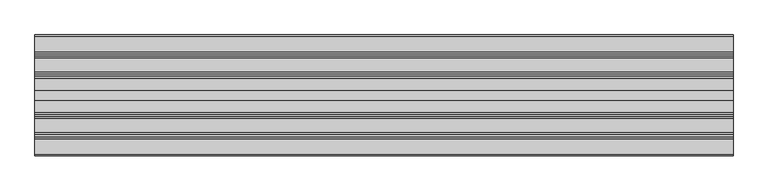
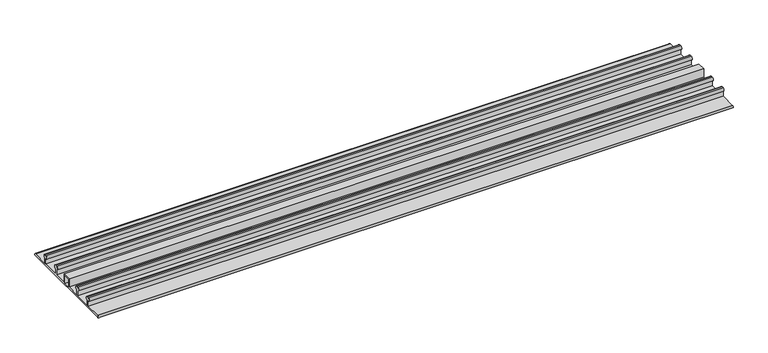
"""IFC4 building model written with IfcOpenShell, lengths in millimetres: proxy geometry, TN_ПВХ_ТПО_Гидрошпонка ТехноНИКОЛЬ : ПВХ Гидрошпонка ТехноНИКОЛЬ EM-260/20."""

from ifc_helpers import new_model, si_unit, point, frame, frame_2d, origin, place, context, project, spatial, polyline, circle_curve, trimmed, segment, composite_curve, outline, extrude, source, transform, mapped, element, save


def specialty_equipment_cb169843(model_context):
    return source(origin(), model_context, "Body", "SweptSolid", [
        extrude(outline(composite_curve([segment(polyline([(127.5, 0.0), (-127.5, 0.0)]), True, "CONTINUOUS"), segment(trimmed(circle_curve(frame_2d((-127.5, 2.5)), 2.5), [point((-127.5, 0.0))], [point((-127.5, 5.0))], False, "CARTESIAN"), True, "CONTINUOUS"), segment(polyline([(-127.5, 5.0), (-88.7123259, 5.0), (-88.7123259, 18.0)]), True, "CONTINUOUS"), segment(trimmed(circle_curve(frame_2d((-88.7123259, 22.0)), 4.0), [point((-88.7123259, 18.0))], [point((-88.7123259, 26.0))], False, "CARTESIAN"), True, "CONTINUOUS"), segment(polyline([(-88.7123259, 26.0), (-84.6210074, 26.0)]), True, "CONTINUOUS"), segment(trimmed(circle_curve(frame_2d((-84.6210074, 22.0)), 4.0), [point((-84.6210074, 26.0))], [point((-84.6210074, 18.0))], False, "CARTESIAN"), True, "CONTINUOUS"), segment(polyline([(-84.6210074, 18.0), (-84.6210074, 5.0), (-45.3789926, 5.0), (-45.3789926, 18.0)]), True, "CONTINUOUS"), segment(trimmed(circle_curve(frame_2d((-45.3789926, 22.0)), 4.0), [point((-45.3789926, 18.0))], [point((-45.3789926, 26.0))], False, "CARTESIAN"), True, "CONTINUOUS"), segment(polyline([(-45.3789926, 26.0), (-41.2876741, 26.0)]), True, "CONTINUOUS"), segment(trimmed(circle_curve(frame_2d((-41.2876741, 22.0)), 4.0), [point((-41.2876741, 26.0))], [point((-41.2876741, 18.0))], False, "CARTESIAN"), True, "CONTINUOUS"), segment(polyline([(-41.2876741, 18.0), (-41.2876741, 5.0), (-10.0, 5.0), (-10.0, 26.0), (10.0, 26.0), (10.0, 5.0), (41.2876741, 5.0), (41.2876741, 18.0)]), True, "CONTINUOUS"), segment(trimmed(circle_curve(frame_2d((41.2876741, 22.0)), 4.0), [point((41.2876741, 18.0))], [point((41.2876741, 26.0))], False, "CARTESIAN"), True, "CONTINUOUS"), segment(polyline([(41.2876741, 26.0), (45.3789926, 26.0)]), True, "CONTINUOUS"), segment(trimmed(circle_curve(frame_2d((45.3789926, 22.0)), 4.0), [point((45.3789926, 26.0))], [point((45.3789926, 18.0))], False, "CARTESIAN"), True, "CONTINUOUS"), segment(polyline([(45.3789926, 18.0), (45.3789926, 5.0), (84.6210074, 5.0), (84.6210074, 18.0)]), True, "CONTINUOUS"), segment(trimmed(circle_curve(frame_2d((84.6210074, 22.0)), 4.0), [point((84.6210074, 18.0))], [point((84.6210074, 26.0))], False, "CARTESIAN"), True, "CONTINUOUS"), segment(polyline([(84.6210074, 26.0), (88.7123259, 26.0)]), True, "CONTINUOUS"), segment(trimmed(circle_curve(frame_2d((88.7123259, 22.0)), 4.0), [point((88.7123259, 26.0))], [point((88.7123259, 18.0))], False, "CARTESIAN"), True, "CONTINUOUS"), segment(polyline([(88.7123259, 18.0), (88.7123259, 5.0), (127.5, 5.0)]), True, "CONTINUOUS"), segment(trimmed(circle_curve(frame_2d((127.5, 2.5)), 2.5), [point((127.5, 5.0))], [point((127.5, 0.0))], False, "CARTESIAN"), True, "CONTINUOUS")], self_intersect=False), holes=[polyline([(-7.0213922, 23.012356), (-7.0213922, 3.7793951), (7.0213922, 3.7793951), (7.0213922, 23.012356), (-7.0213922, 23.012356)])]), frame((0.0, 0.0, 0.0), z_axis=(1.0, 0.0, 0.0), x_axis=(0.0, 1.0, 0.0)), (0.0, 0.0, 1.0), 1500.0),
    ])


if __name__ == "__main__":
    model = new_model("IFC4")
    model_context = context("Model", 3, world=origin())
    ifc_project = project(units=[si_unit("LENGTHUNIT", "METRE", prefix="MILLI")], contexts=[model_context])
    site = spatial("IfcSite", under=ifc_project)
    building = spatial("IfcBuilding", under=site)
    placement = place(None, origin())
    specialty_equipment_shape = specialty_equipment_cb169843(model_context)
    element("IfcBuildingElementProxy", 1, Name="TN_ПВХ_ТПО_Гидрошпонка ТехноНИКОЛЬ : ПВХ Гидрошпонка ТехноНИКОЛЬ EM-260/20", ObjectType="TN_ПВХ_ТПО_Гидрошпонка ТехноНИКОЛЬ : ПВХ Гидрошпонка ТехноНИКОЛЬ EM-260/20", at=placement, inside=building, context=model_context, shape_type="MappedRepresentation", body=[
        mapped(specialty_equipment_shape, transform((0.0, 0.0, 0.0), x_axis=(1.0, 0.0, 0.0), y_axis=(0.0, 1.0, 0.0), z_axis=(0.0, 0.0, 1.0))),
    ])
    save(model, "model.ifc")

# Revit data of these elements
# Type "TN_ПВХ_ТПО_Гидрошпонка ТехноНИКОЛЬ : ПВХ Гидрошпонка ТехноНИКОЛЬ EM-260/20"
#   Description = "Опалубочная деформационная ПВХ гидрошпонка. Ширина деформационного узла 20 мм. Применяется для герметизации деформационных швов при строительстве заглубленных и подземных сооружений"
#   Type Comments = "п.м."
#   Manufacturer = "ТехноНИКОЛЬ"
#   URL = "https://shop.tn.ru/pvh-gidroshponka-em-260-20-10-m-rul"
#   ADSK_Примечание = ""
#   ADSK_Обозначение [instance default] = "ТехноНИКОЛЬ"
#   ADSK_Наименование = "ПВХ Гидрошпонка ТехноНИКОЛЬ EM-260/20, 10м/рул"
#   ADSK_Масса_Текст = ""
#   ADSK_Марка = ""
#   ADSK_Код изделия = "499887"
#   ADSK_Завод-изготовитель [instance default] = "ТехноНИКОЛЬ"
#   ADSK_Единица измерения [instance default] = "п.м."
#   ADSK_Группирование = "Гидрошпонки"
#   ADSK_URL страницы изделия = "https://shop.tn.ru/pvh-gidroshponka-em-260-20-10-m-rul"
#   ADSK_URL документации изделия = "https://nav.tn.ru/upload/iblock/67f/Katalog-i-rekomendatsii-po-primeneniyu_Gidroshponki-TEKHNONIKOL.PDF"
#   built-in parameter 1001306 [instance default] = 3.28084 (stored number, unit not read)
#   ADSK_Размер_Длина [instance default] = 1000 mm
#   ADSK_Количество [instance default] = 1
#   ПВХ_ТПО Гидрошпонка ТехноНИКОЛЬ EC-320-4 = no
#   ПВХ Гидрошпонка ТехноНИКОЛЬ IM-260/50 = no
#   ПВХ Гидрошпонка ТехноНИКОЛЬ IM-240/20 = no
#   ПВХ Гидрошпонка ТехноНИКОЛЬ IC-240-6 = no
#   ПВХ Гидрошпонка ТехноНИКОЛЬ IC-125-2SP = no
#   ПВХ Гидрошпонка ТехноНИКОЛЬ EM-260/50 = no
#   ПВХ Гидрошпонка ТехноНИКОЛЬ EM-260/20 = yes
#   ПВХ Гидрошпонка ТехноНИКОЛЬ EC-320-4 = no
#   ПВХ Гидрошпонка ТехноНИКОЛЬ EC-220-3 = no
#   ПВХ_ТПО Гидрошпонка ТехноНИКОЛЬ EC-220-3 = no
#   ПВХ Гидрошпонка ТехноНИКОЛЬ IC-240-2 = no
#   Материал = TN_ПВХ_Черный
#   Default Elevation = 0
# Element 1 (IfcBuildingElementProxy, "TN_ПВХ_ТПО_Гидрошпонка ТехноНИКОЛЬ : ПВХ Гидрошпонка ТехноНИКОЛЬ EM-260/20")
#   built-in parameter 1001306 = 4.92126 (stored number, unit not read)
#   ADSK_Размер_Длина = 1500 mm
#   ADSK_Количество = 1.5
#   Materials on its faces: "TN_ПВХ_Черный"
# Materials
#   "TN_ПВХ_Черный": class "Типовые", colour RGB 48 48 48, transparency 0, Cost = 0
